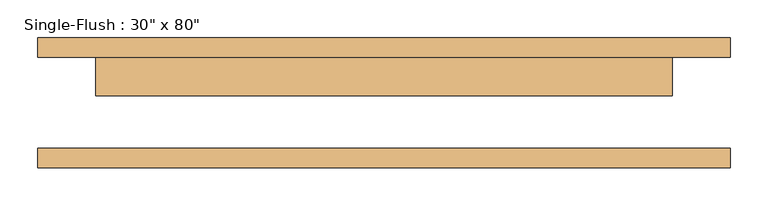
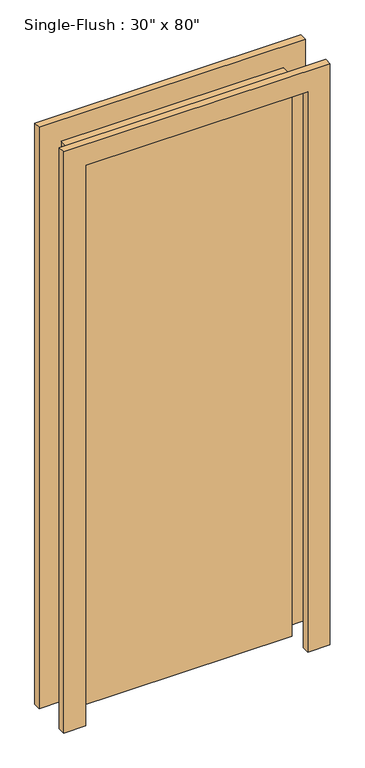
"""IFC4 building model written with IfcOpenShell, lengths in millimetres: door geometry."""

from ifc_helpers import new_model, si_unit, frame, origin, origin_with_axes, place, context, project, spatial, polyline, outline, extrude, source, transform, mapped, element, save


def door_1e92232a(model_context):
    return source(origin(), model_context, "Body", "SweptSolid", [
        extrude(outline(polyline([(2108.2, -457.2), (0.0, -457.2), (0.0, -381.0), (2032.0, -381.0), (2032.0, 381.0), (0.0, 381.0), (0.0, 457.2), (2108.2, 457.2), (2108.2, -457.2)])), frame((0.0, 60.325, 0.0), z_axis=(0.0, 1.0, 0.0), x_axis=(0.0, 0.0, 1.0)), (0.0, 0.0, 1.0), 25.4),
        extrude(outline(polyline([(2108.2, 457.2), (2108.2, -457.2), (0.0, -457.2), (0.0, -381.0), (2032.0, -381.0), (2032.0, 381.0), (0.0, 381.0), (0.0, 457.2), (2108.2, 457.2)])), frame((0.0, -85.725, 0.0), z_axis=(0.0, 1.0, 0.0), x_axis=(0.0, 0.0, 1.0)), (0.0, 0.0, 1.0), 25.4),
        extrude(outline(polyline([(381.0, 9.525), (-381.0, 9.525), (-381.0, 60.325), (381.0, 60.325), (381.0, 9.525)])), origin_with_axes(), (0.0, 0.0, 1.0), 2032.0),
    ])


if __name__ == "__main__":
    model = new_model("IFC4")
    model_context = context("Model", 3, world=origin())
    ifc_project = project(units=[si_unit("LENGTHUNIT", "METRE", prefix="MILLI")], contexts=[model_context])
    site = spatial("IfcSite", under=ifc_project)
    building = spatial("IfcBuilding", under=site)
    placement = place(None, origin())
    door_shape = door_1e92232a(model_context)
    element("IfcDoor", 1, ObjectType="Single-Flush : 30\" x 80\"", at=placement, inside=building, context=model_context, shape_type="MappedRepresentation", body=[
        mapped(door_shape, transform((0.0, 0.0, 0.0), x_axis=(1.0, 0.0, 0.0), y_axis=(0.0, 1.0, 0.0), z_axis=(0.0, 0.0, 1.0))),
    ])
    save(model, "model.ifc")

# Revit data of these elements
# Type "Single-Flush : 30\" x 80\""
#   Type Mark = "5"
#   Assembly Code = "C1020"
#   Thickness = 0' - 2"
#   Height = 6' - 8"
#   Trim Projection Ext = 0' - 1"
#   Trim Projection Int = 0' - 1"
#   Trim Width = 0' - 3"
#   Width = 2' - 6"
#   Door Material = none
#   Frame Material = none
#   Function = (empty or 0)
#   Wall Closure = (empty or 0)
